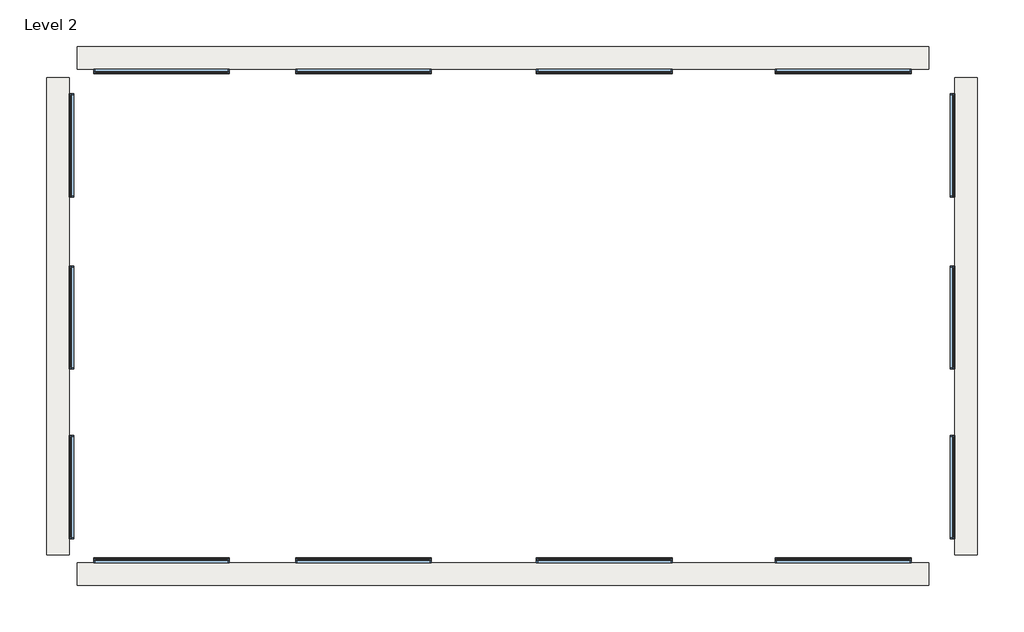
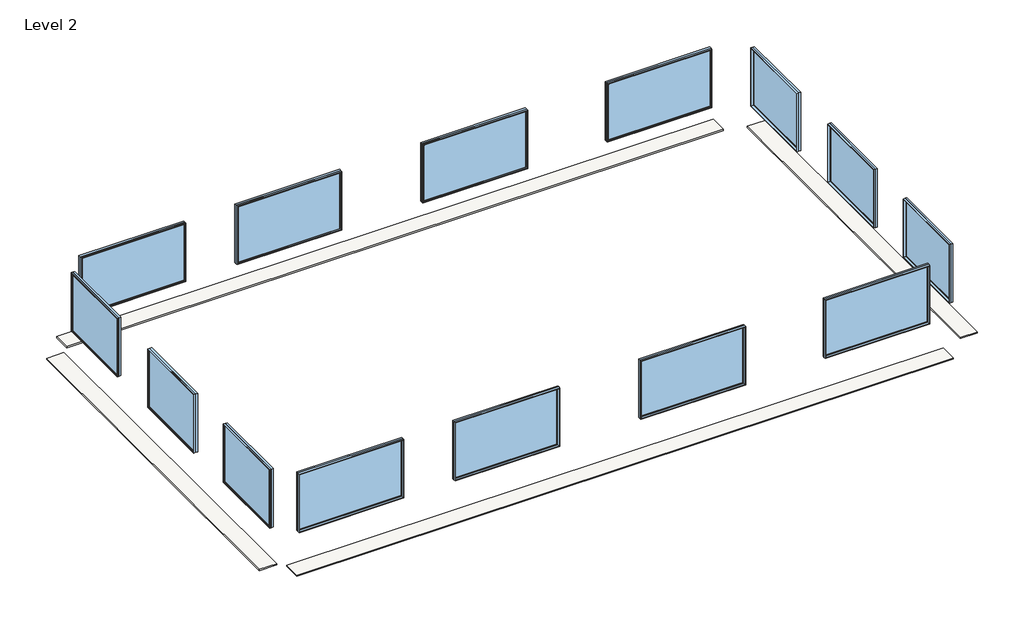
# One storey: 14 windows, 4 roofs.
"""IFC4 building model written with IfcOpenShell, lengths in millimetres."""

import ifcopenshell
import ifcopenshell.guid

model = None  # the IFC model being written
_history = None  # IfcOwnerHistory: only IFC2X3 demands one
_inside = {}  # id of a spatial element -> (the spatial element, [elements in it])
_under = {}  # id of a project, library or spatial element -> (it, [spatial elements below it])
_declared = {}  # id of a project -> (the project, [libraries it declares])
_typed = {}  # id of a type object -> (the type object, [elements of that type])
_made_of = {}  # id of a material, layer set ... -> (it, [elements and type objects made of it])


def new_model(schema):
    """Start an empty IFC model of exactly this schema.

    Asked for "IFC4X3", IfcOpenShell would pick the latest addendum, in which some entities
    have other attributes; the version numbers below select the first issue.
    IFC2X3 requires an IfcOwnerHistory on every rooted entity: one is made here for all.
    """
    global model, _history
    if schema == "IFC4X3":
        model = ifcopenshell.file(schema_version=(4, 3, 0, 0))
    else:
        model = ifcopenshell.file(schema=schema)
    _inside.clear()
    _under.clear()
    _declared.clear()
    _typed.clear()
    _made_of.clear()
    _history = None
    if model.schema == "IFC2X3":
        org = make("IfcOrganization", Name="unknown")
        user = make(
            "IfcPersonAndOrganization",
            ThePerson=make("IfcPerson", FamilyName="unknown"),
            TheOrganization=org,
        )
        app = make(
            "IfcApplication",
            ApplicationDeveloper=org,
            Version="unknown",
            ApplicationFullName="unknown",
            ApplicationIdentifier="unknown",
        )
        _history = make(
            "IfcOwnerHistory",
            OwningUser=user,
            OwningApplication=app,
            ChangeAction="ADDED",
            CreationDate=0,
        )
    return model


def make(cls, **values):
    """One entity of the class cls with the attributes given. An attribute that is None is left unset."""
    return model.create_entity(
        cls, **{name: value for name, value in values.items() if value is not None}
    )


def rooted(cls, **values):
    """An entity with a GlobalId (a new one), such as an element, a storey or a relation."""
    return make(cls, GlobalId=ifcopenshell.guid.new(), OwnerHistory=_history, **values)


def si_unit(unit_type, name, prefix=None):
    """IfcSIUnit, for example si_unit("LENGTHUNIT", "METRE", prefix="MILLI")."""
    return make("IfcSIUnit", UnitType=unit_type, Prefix=prefix, Name=name)


def assignment(units):
    """IfcUnitAssignment: the units of a project."""
    return None if units is None else make("IfcUnitAssignment", Units=units)


def point(xyz):
    """IfcCartesianPoint."""
    return None if xyz is None else make("IfcCartesianPoint", Coordinates=xyz)


def direction(xyz):
    """IfcDirection."""
    return None if xyz is None else make("IfcDirection", DirectionRatios=xyz)


def frame(location, z_axis=None, x_axis=None):
    """IfcAxis2Placement3D, a coordinate frame: its origin and axes. An axis left out is left unset."""
    return make(
        "IfcAxis2Placement3D",
        Location=point(location),
        Axis=direction(z_axis),
        RefDirection=direction(x_axis),
    )


def origin():
    """The frame at (0, 0, 0) with its axes left unset."""
    return frame((0.0, 0.0, 0.0))


def place(relative_to, where):
    """IfcLocalPlacement: puts the frame where relative to a parent placement (None: the world)."""
    return make(
        "IfcLocalPlacement", PlacementRelTo=relative_to, RelativePlacement=where
    )


def context(
    kind, dimensions, precision=None, world=None, true_north=None, identifier=None
):
    """IfcGeometricRepresentationContext, for example the 3D "Model" context."""
    return make(
        "IfcGeometricRepresentationContext",
        ContextIdentifier=identifier,
        ContextType=kind,
        CoordinateSpaceDimension=dimensions,
        Precision=precision,
        WorldCoordinateSystem=world,
        TrueNorth=true_north,
    )


def project(units=None, contexts=None):
    """IfcProject with its units and contexts."""
    return rooted(
        "IfcProject",
        Name="project",
        RepresentationContexts=contexts,
        UnitsInContext=assignment(units),
    )


def spatial(cls, under=None, at=None, **own):
    """A site, building, storey or space (cls), placed at a placement, below another one or the project."""
    s = rooted(cls, ObjectPlacement=at, **own)
    if under is not None:
        _under.setdefault(under.id(), (under, []))[1].append(s)
    return s


def polyline(points):
    """IfcPolyline through the points."""
    return make("IfcPolyline", Points=[point(p) for p in points])


def outline(outer, holes=None, kind="AREA"):
    """IfcArbitraryClosedProfileDef: a profile drawn as a closed curve; with holes, ...WithVoids."""
    if holes is None:
        return make("IfcArbitraryClosedProfileDef", ProfileType=kind, OuterCurve=outer)
    return make(
        "IfcArbitraryProfileDefWithVoids",
        ProfileType=kind,
        OuterCurve=outer,
        InnerCurves=holes,
    )


def extrude(swept, where, along, depth):
    """IfcExtrudedAreaSolid: the profile swept, set in the frame where, extruded along a direction by depth."""
    return make(
        "IfcExtrudedAreaSolid",
        SweptArea=swept,
        Position=where,
        ExtrudedDirection=direction(along),
        Depth=depth,
    )


def shape(context_of_items, identifier, shape_type, items):
    """IfcShapeRepresentation: the items that make up one representation, for example the "Body"."""
    return make(
        "IfcShapeRepresentation",
        ContextOfItems=context_of_items,
        RepresentationIdentifier=identifier,
        RepresentationType=shape_type,
        Items=items,
    )


def source(mapping_origin, context_of_items, identifier, shape_type, items):
    """IfcRepresentationMap: a shape defined once, which mapped items show again and again."""
    return make(
        "IfcRepresentationMap",
        MappingOrigin=mapping_origin,
        MappedRepresentation=shape(context_of_items, identifier, shape_type, items),
    )


def transform(
    local_origin,
    x_axis=None,
    y_axis=None,
    z_axis=None,
    scale=None,
    scale2=None,
    scale3=None,
    uniform=True,
):
    """IfcCartesianTransformationOperator3D, or its non-uniform kind. x_axis, y_axis, z_axis: its Axis1, 2, 3."""
    if uniform:
        return make(
            "IfcCartesianTransformationOperator3D",
            Axis1=direction(x_axis),
            Axis2=direction(y_axis),
            LocalOrigin=point(local_origin),
            Scale=scale,
            Axis3=direction(z_axis),
        )
    return make(
        "IfcCartesianTransformationOperator3DnonUniform",
        Axis1=direction(x_axis),
        Axis2=direction(y_axis),
        LocalOrigin=point(local_origin),
        Scale=scale,
        Axis3=direction(z_axis),
        Scale2=scale2,
        Scale3=scale3,
    )


def mapped(mapping_source, mapping_target):
    """IfcMappedItem: shows the shape of a source again, moved by a transform."""
    return make(
        "IfcMappedItem", MappingSource=mapping_source, MappingTarget=mapping_target
    )


def made_of(thing, what):
    """Note that an element or type object is made of a material, layer set ...; save() writes the relation."""
    if what is not None:
        _made_of.setdefault(what.id(), (what, []))[1].append(thing)
    return thing


def element(
    cls,
    number,
    at=None,
    inside=None,
    cuts=None,
    type_object=None,
    material=None,
    context=None,
    identifier="Body",
    shape_type=None,
    held_by="IfcProductDefinitionShape",
    body=None,
    shapes=None,
    **own,
):
    """One element of the class cls, such as IfcWall. Its Tag is "e" and its number.

    at: its placement. inside: the storey or other place that contains it. cuts: it is an
    opening in that element (IfcRelVoidsElement). A single representation is given by context,
    identifier, shape_type and body (its items); several are given by shapes. held_by: the class
    of the entity that holds the representations. save() writes the other relations.
    """
    e = rooted(cls, Tag="e%d" % number, ObjectPlacement=at, **own)
    if body is not None:
        shapes = [shape(context, identifier, shape_type, body)]
    if shapes is not None:
        e.Representation = make(held_by, Representations=shapes)
    if inside is not None:
        _inside.setdefault(inside.id(), (inside, []))[1].append(e)
    if cuts is not None:
        rooted(
            "IfcRelVoidsElement", RelatingBuildingElement=cuts, RelatedOpeningElement=e
        )
    if type_object is not None:
        _typed.setdefault(type_object.id(), (type_object, []))[1].append(e)
    return made_of(e, material)


def aggregate(whole, parts):
    """IfcRelAggregates: a whole, such as a stair, and the parts it consists of."""
    return rooted("IfcRelAggregates", RelatingObject=whole, RelatedObjects=parts)


def save(model, path):
    """Write the relations noted so far, then the file.

    IfcRelAggregates (storeys below a building ...), IfcRelContainedInSpatialStructure (elements
    in a storey), IfcRelDefinesByType, IfcRelAssociatesMaterial and IfcRelDeclares: one each for
    every whole, place, type object, material and project.
    """
    for whole, parts in _under.values():
        aggregate(whole, parts)
    for where, things in _inside.values():
        rooted(
            "IfcRelContainedInSpatialStructure",
            RelatedElements=things,
            RelatingStructure=where,
        )
    for kind, things in _typed.values():
        rooted("IfcRelDefinesByType", RelatedObjects=things, RelatingType=kind)
    for what, things in _made_of.values():
        rooted("IfcRelAssociatesMaterial", RelatedObjects=things, RelatingMaterial=what)
    for by, libraries in _declared.values():
        rooted("IfcRelDeclares", RelatingContext=by, RelatedDefinitions=libraries)
    model.write(path)


def m_fixed_2500x_4228mm_fd5e51e7(model_context):
    return source(origin(), model_context, "Body", "SweptSolid", [
        extrude(outline(polyline([(-2050.8, 54.2), (2050.8, 54.2), (2050.8, 42.2), (-2050.8, 42.2), (-2050.8, 54.2)])), frame((0.0, 0.0, 368.0), z_axis=(0.0, 0.0, 1.0), x_axis=(1.0, 0.0, 0.0)), (0.0, 0.0, 1.0), 2374.0),
        extrude(outline(polyline([(2786.0, -2094.8), (324.0, -2094.8), (324.0, 2094.8), (2786.0, 2094.8), (2786.0, -2094.8)]), holes=[polyline([(2742.0, -2050.8), (2742.0, 2050.8), (368.0, 2050.8), (368.0, -2050.8), (2742.0, -2050.8)])]), frame((0.0, 26.2, 0.0), z_axis=(0.0, 1.0, 0.0), x_axis=(0.0, 0.0, 1.0)), (0.0, 0.0, 1.0), 44.0),
        extrude(outline(polyline([(2805.0, -2113.8), (305.0, -2113.8), (305.0, 2113.8), (2805.0, 2113.8), (2805.0, -2113.8)]), holes=[polyline([(2786.0, -2094.8), (2786.0, 2094.8), (324.0, 2094.8), (324.0, -2094.8), (2786.0, -2094.8)])]), frame((0.0, 26.2, 0.0), z_axis=(0.0, 1.0, 0.0), x_axis=(0.0, 0.0, 1.0)), (0.0, 0.0, 1.0), 63.0),
        extrude(outline(polyline([(2805.0, -2113.8), (305.0, -2113.8), (305.0, 2113.8), (2805.0, 2113.8), (2805.0, -2113.8)]), holes=[polyline([(2773.0, -2081.8), (2773.0, 2081.8), (337.0, 2081.8), (337.0, -2081.8), (2773.0, -2081.8)])]), frame((0.0, -63.2, 0.0), z_axis=(0.0, 1.0, 0.0), x_axis=(0.0, 0.0, 1.0)), (0.0, 0.0, 1.0), 89.4),
    ])


def m_fixed_2500x_4228mm_f14c179f(model_context):
    return source(origin(), model_context, "Body", "SweptSolid", [
        extrude(outline(polyline([(-2050.8, -54.2), (-2050.8, -42.2), (2050.8, -42.2), (2050.8, -54.2), (-2050.8, -54.2)])), frame((0.0, 0.0, 368.0), z_axis=(0.0, 0.0, 1.0), x_axis=(1.0, 0.0, 0.0)), (0.0, 0.0, 1.0), 2374.0),
        extrude(outline(polyline([(2786.0, -2094.8), (324.0, -2094.8), (324.0, 2094.8), (2786.0, 2094.8), (2786.0, -2094.8)]), holes=[polyline([(2742.0, -2050.8), (2742.0, 2050.8), (368.0, 2050.8), (368.0, -2050.8), (2742.0, -2050.8)])]), frame((0.0, -70.2, 0.0), z_axis=(0.0, 1.0, 0.0), x_axis=(0.0, 0.0, 1.0)), (0.0, 0.0, 1.0), 44.0),
        extrude(outline(polyline([(2805.0, -2113.8), (305.0, -2113.8), (305.0, 2113.8), (2805.0, 2113.8), (2805.0, -2113.8)]), holes=[polyline([(2786.0, -2094.8), (2786.0, 2094.8), (324.0, 2094.8), (324.0, -2094.8), (2786.0, -2094.8)])]), frame((0.0, -89.2, 0.0), z_axis=(0.0, 1.0, 0.0), x_axis=(0.0, 0.0, 1.0)), (0.0, 0.0, 1.0), 63.0),
        extrude(outline(polyline([(2805.0, -2113.8), (305.0, -2113.8), (305.0, 2113.8), (2805.0, 2113.8), (2805.0, -2113.8)]), holes=[polyline([(2773.0, -2081.8), (2773.0, 2081.8), (337.0, 2081.8), (337.0, -2081.8), (2773.0, -2081.8)])]), frame((0.0, -26.2, 0.0), z_axis=(0.0, 1.0, 0.0), x_axis=(0.0, 0.0, 1.0)), (0.0, 0.0, 1.0), 89.4),
    ])


def m_fixed_2500x_3220mm_df94f4d0(model_context):
    return source(origin(), model_context, "Body", "SweptSolid", [
        extrude(outline(polyline([(-1546.8, 54.2), (1546.8, 54.2), (1546.8, 42.2), (-1546.8, 42.2), (-1546.8, 54.2)])), frame((0.0, 0.0, 368.0), z_axis=(0.0, 0.0, 1.0), x_axis=(1.0, 0.0, 0.0)), (0.0, 0.0, 1.0), 2374.0),
        extrude(outline(polyline([(2786.0, -1590.8), (324.0, -1590.8), (324.0, 1590.8), (2786.0, 1590.8), (2786.0, -1590.8)]), holes=[polyline([(2742.0, -1546.8), (2742.0, 1546.8), (368.0, 1546.8), (368.0, -1546.8), (2742.0, -1546.8)])]), frame((0.0, 26.2, 0.0), z_axis=(0.0, 1.0, 0.0), x_axis=(0.0, 0.0, 1.0)), (0.0, 0.0, 1.0), 44.0),
        extrude(outline(polyline([(2805.0, -1609.8), (305.0, -1609.8), (305.0, 1609.8), (2805.0, 1609.8), (2805.0, -1609.8)]), holes=[polyline([(2786.0, -1590.8), (2786.0, 1590.8), (324.0, 1590.8), (324.0, -1590.8), (2786.0, -1590.8)])]), frame((0.0, 26.2, 0.0), z_axis=(0.0, 1.0, 0.0), x_axis=(0.0, 0.0, 1.0)), (0.0, 0.0, 1.0), 63.0),
        extrude(outline(polyline([(2805.0, -1609.8), (305.0, -1609.8), (305.0, 1609.8), (2805.0, 1609.8), (2805.0, -1609.8)]), holes=[polyline([(2773.0, -1577.8), (2773.0, 1577.8), (337.0, 1577.8), (337.0, -1577.8), (2773.0, -1577.8)])]), frame((0.0, -63.2, 0.0), z_axis=(0.0, 1.0, 0.0), x_axis=(0.0, 0.0, 1.0)), (0.0, 0.0, 1.0), 89.4),
    ])


def m_fixed_2500x_3220mm_8b997f8c(model_context):
    return source(origin(), model_context, "Body", "SweptSolid", [
        extrude(outline(polyline([(-1546.8, -54.2), (-1546.8, -42.2), (1546.8, -42.2), (1546.8, -54.2), (-1546.8, -54.2)])), frame((0.0, 0.0, 368.0), z_axis=(0.0, 0.0, 1.0), x_axis=(1.0, 0.0, 0.0)), (0.0, 0.0, 1.0), 2374.0),
        extrude(outline(polyline([(2786.0, -1590.8), (324.0, -1590.8), (324.0, 1590.8), (2786.0, 1590.8), (2786.0, -1590.8)]), holes=[polyline([(2742.0, -1546.8), (2742.0, 1546.8), (368.0, 1546.8), (368.0, -1546.8), (2742.0, -1546.8)])]), frame((0.0, -70.2, 0.0), z_axis=(0.0, 1.0, 0.0), x_axis=(0.0, 0.0, 1.0)), (0.0, 0.0, 1.0), 44.0),
        extrude(outline(polyline([(2805.0, -1609.8), (305.0, -1609.8), (305.0, 1609.8), (2805.0, 1609.8), (2805.0, -1609.8)]), holes=[polyline([(2786.0, -1590.8), (2786.0, 1590.8), (324.0, 1590.8), (324.0, -1590.8), (2786.0, -1590.8)])]), frame((0.0, -89.2, 0.0), z_axis=(0.0, 1.0, 0.0), x_axis=(0.0, 0.0, 1.0)), (0.0, 0.0, 1.0), 63.0),
        extrude(outline(polyline([(2805.0, -1609.8), (305.0, -1609.8), (305.0, 1609.8), (2805.0, 1609.8), (2805.0, -1609.8)]), holes=[polyline([(2773.0, -1577.8), (2773.0, 1577.8), (337.0, 1577.8), (337.0, -1577.8), (2773.0, -1577.8)])]), frame((0.0, -26.2, 0.0), z_axis=(0.0, 1.0, 0.0), x_axis=(0.0, 0.0, 1.0)), (0.0, 0.0, 1.0), 89.4),
    ])


model = new_model("IFC4")

# Units and contexts
model_context = context("Model", 3, world=origin())
ifc_project = project(units=[si_unit("LENGTHUNIT", "METRE", prefix="MILLI")], contexts=[model_context])

# Site, building, storey
site = spatial("IfcSite", under=ifc_project)
building = spatial("IfcBuilding", under=site)
storey = spatial("IfcBuildingStorey", under=building, Name="Level 2", Elevation=3962.4)

# Roofs
placement = place(None, origin())
element("IfcRoof", 1, ObjectType="Shading devices - 50mm", at=placement, inside=storey, context=model_context, shape_type="SweptSolid", body=[
    extrude(outline(polyline([(1746.464681, -4095.4197783), (28246.464681, -4095.4197783), (28246.464681, -4795.4197783), (1746.464681, -4795.4197783), (1746.464681, -4095.4197783)])), frame((0.0, 0.0, 3602.4), z_axis=(0.0, 0.0, 1.0), x_axis=(1.0, 0.0, 0.0)), (0.0, 0.0, 1.0), 50.0),
])
element("IfcRoof", 2, ObjectType="Shading devices - 50mm", at=placement, inside=storey, context=model_context, shape_type="SweptSolid", body=[
    extrude(outline(polyline([(29068.464681, 11030.5802217), (29768.464681, 11030.5802217), (29768.464681, -3843.0197783), (29068.464681, -3843.0197783), (29068.464681, 11030.5802217)])), frame((0.0, 0.0, 3602.4), z_axis=(0.0, 0.0, 1.0), x_axis=(1.0, 0.0, 0.0)), (0.0, 0.0, 1.0), 50.0),
])
element("IfcRoof", 3, ObjectType="Shading devices - 50mm", at=placement, inside=storey, context=model_context, shape_type="SweptSolid", body=[
    extrude(outline(polyline([(28246.464681, 11296.9802217), (1746.464681, 11296.9802217), (1746.464681, 11996.9802217), (28246.464681, 11996.9802217), (28246.464681, 11296.9802217)])), frame((0.0, 0.0, 3602.4), z_axis=(0.0, 0.0, 1.0), x_axis=(1.0, 0.0, 0.0)), (0.0, 0.0, 1.0), 50.0),
])
element("IfcRoof", 4, ObjectType="Shading devices - 50mm", at=placement, inside=storey, context=model_context, shape_type="SweptSolid", body=[
    extrude(outline(polyline([(784.064681, 11030.5802217), (1484.064681, 11030.5802217), (1484.064681, -3843.0197783), (784.064681, -3843.0197783), (784.064681, 11030.5802217)])), frame((0.0, 0.0, 3602.4), z_axis=(0.0, 0.0, 1.0), x_axis=(1.0, 0.0, 0.0)), (0.0, 0.0, 1.0), 50.0),
])

# Windows
m_fixed_2500x_4228mm_shape = m_fixed_2500x_4228mm_fd5e51e7(model_context)
element("IfcWindow", 5, ObjectType="M_Fixed : 2500X 4228mm", at=placement, inside=storey, context=model_context, shape_type="MappedRepresentation", body=[
    mapped(m_fixed_2500x_4228mm_shape, transform((4360.264681, 11233.7802217, 4557.4), x_axis=(-1.0, 0.0, 0.0), y_axis=(0.0, -1.0, 0.0), z_axis=(0.0, 0.0, 1.0))),
])
element("IfcWindow", 6, ObjectType="M_Fixed : 2500X 4228mm", at=placement, inside=storey, context=model_context, shape_type="MappedRepresentation", body=[
    mapped(m_fixed_2500x_4228mm_shape, transform((10652.264681, 11233.7802217, 4557.4), x_axis=(-1.0, 0.0, 0.0), y_axis=(0.0, -1.0, 0.0), z_axis=(0.0, 0.0, 1.0))),
])
element("IfcWindow", 7, ObjectType="M_Fixed : 2500X 4228mm", at=placement, inside=storey, context=model_context, shape_type="MappedRepresentation", body=[
    mapped(m_fixed_2500x_4228mm_shape, transform((18152.264681, 11233.7802217, 4557.4), x_axis=(-1.0, 0.0, 0.0), y_axis=(0.0, -1.0, 0.0), z_axis=(0.0, 0.0, 1.0))),
])
element("IfcWindow", 8, ObjectType="M_Fixed : 2500X 4228mm", at=placement, inside=storey, context=model_context, shape_type="MappedRepresentation", body=[
    mapped(m_fixed_2500x_4228mm_shape, transform((25592.264681, 11233.7802217, 4557.4), x_axis=(-1.0, 0.0, 0.0), y_axis=(0.0, -1.0, 0.0), z_axis=(0.0, 0.0, 1.0))),
])
m_fixed_2500x_4228mm_2_shape = m_fixed_2500x_4228mm_f14c179f(model_context)
element("IfcWindow", 9, ObjectType="M_Fixed : 2500X 4228mm", at=placement, inside=storey, context=model_context, shape_type="MappedRepresentation", body=[
    mapped(m_fixed_2500x_4228mm_2_shape, transform((4360.264681, -4032.2197783, 4557.4), x_axis=(-1.0, 0.0, 0.0), y_axis=(0.0, -1.0, 0.0), z_axis=(0.0, 0.0, 1.0))),
])
element("IfcWindow", 10, ObjectType="M_Fixed : 2500X 4228mm", at=placement, inside=storey, context=model_context, shape_type="MappedRepresentation", body=[
    mapped(m_fixed_2500x_4228mm_2_shape, transform((10652.264681, -4032.2197783, 4557.4), x_axis=(-1.0, 0.0, 0.0), y_axis=(0.0, -1.0, 0.0), z_axis=(0.0, 0.0, 1.0))),
])
element("IfcWindow", 11, ObjectType="M_Fixed : 2500X 4228mm", at=placement, inside=storey, context=model_context, shape_type="MappedRepresentation", body=[
    mapped(m_fixed_2500x_4228mm_2_shape, transform((18152.264681, -4032.2197783, 4557.4), x_axis=(-1.0, 0.0, 0.0), y_axis=(0.0, -1.0, 0.0), z_axis=(0.0, 0.0, 1.0))),
])
element("IfcWindow", 12, ObjectType="M_Fixed : 2500X 4228mm", at=placement, inside=storey, context=model_context, shape_type="MappedRepresentation", body=[
    mapped(m_fixed_2500x_4228mm_2_shape, transform((25592.264681, -4032.2197783, 4557.4), x_axis=(-1.0, 0.0, 0.0), y_axis=(0.0, -1.0, 0.0), z_axis=(0.0, 0.0, 1.0))),
])
m_fixed_2500x_3220mm_shape = m_fixed_2500x_3220mm_df94f4d0(model_context)
element("IfcWindow", 13, ObjectType="M_Fixed : 2500x 3220mm", at=placement, inside=storey, context=model_context, shape_type="MappedRepresentation", body=[
    mapped(m_fixed_2500x_3220mm_shape, transform((1573.264681, 8920.7802217, 4559.8), x_axis=(0.0, 1.0, 0.0), y_axis=(-1.0, 0.0, 0.0), z_axis=(0.0, 0.0, 1.0))),
])
element("IfcWindow", 14, ObjectType="M_Fixed : 2500x 3220mm", at=placement, inside=storey, context=model_context, shape_type="MappedRepresentation", body=[
    mapped(m_fixed_2500x_3220mm_shape, transform((1573.264681, 3552.7802217, 4559.8), x_axis=(0.0, 1.0, 0.0), y_axis=(-1.0, 0.0, 0.0), z_axis=(0.0, 0.0, 1.0))),
])
element("IfcWindow", 15, ObjectType="M_Fixed : 2500x 3220mm", at=placement, inside=storey, context=model_context, shape_type="MappedRepresentation", body=[
    mapped(m_fixed_2500x_3220mm_shape, transform((1573.264681, -1733.2197783, 4559.8), x_axis=(0.0, 1.0, 0.0), y_axis=(-1.0, 0.0, 0.0), z_axis=(0.0, 0.0, 1.0))),
])
m_fixed_2500x_3220mm_2_shape = m_fixed_2500x_3220mm_8b997f8c(model_context)
element("IfcWindow", 16, ObjectType="M_Fixed : 2500x 3220mm", at=placement, inside=storey, context=model_context, shape_type="MappedRepresentation", body=[
    mapped(m_fixed_2500x_3220mm_2_shape, transform((28979.264681, 8920.7802217, 4559.8), x_axis=(0.0, 1.0, 0.0), y_axis=(-1.0, 0.0, 0.0), z_axis=(0.0, 0.0, 1.0))),
])
element("IfcWindow", 17, ObjectType="M_Fixed : 2500x 3220mm", at=placement, inside=storey, context=model_context, shape_type="MappedRepresentation", body=[
    mapped(m_fixed_2500x_3220mm_2_shape, transform((28979.264681, 3552.7802217, 4559.8), x_axis=(0.0, 1.0, 0.0), y_axis=(-1.0, 0.0, 0.0), z_axis=(0.0, 0.0, 1.0))),
])
element("IfcWindow", 18, ObjectType="M_Fixed : 2500x 3220mm", at=placement, inside=storey, context=model_context, shape_type="MappedRepresentation", body=[
    mapped(m_fixed_2500x_3220mm_2_shape, transform((28979.264681, -1733.2197783, 4559.8), x_axis=(0.0, 1.0, 0.0), y_axis=(-1.0, 0.0, 0.0), z_axis=(0.0, 0.0, 1.0))),
])

save(model, "model.ifc")

# Revit data of these elements
# Project information
#   Project Issue Date = "Issue Date"
#   Project Status = "Project Status"
#   Client Name = "Owner"
#   Project Address = "Enter address here"
#   Project Name = "Project Name"
#   Project Number = "Project Number"
# Type "Shading devices - 50mm"
#   Layers, outside or top first: 50 mm no material (function 1)
# Type "M_Fixed : 2500X 4228mm"
#   Type Mark = "25"
#   Height = 2500 mm
#   Default Sill Height = 305 mm
#   Width = 4227.6 mm
#   Window Inset = 19 mm
#   Frame Exterior Material = Sash
#   Frame Interior Material = Sash
#   Glass Pane Material = Glass
#   Sash = Sash
#   Wall Closure = (empty or 0)
# Type "M_Fixed : 2500x 3220mm"
#   Type Mark = "26"
#   Height = 2500 mm
#   Default Sill Height = 305 mm
#   Width = 3219.6 mm
#   Window Inset = 19 mm
#   Frame Exterior Material = Sash
#   Frame Interior Material = Sash
#   Glass Pane Material = Glass
#   Sash = Sash
#   Wall Closure = (empty or 0)
# Elements 1, 2, 3, 4 (IfcRoof, "Shading devices - 50mm")
#   built-in parameter 1001705 = 11.9829 (stored number, unit not read)
#   built-in parameter 1001701 = -1.1811 (stored number, unit not read)
#   built-in parameter 1001710 = 33615
#   Phase Created = New Construction
#   Materials on its faces: "Default Roof"
# Element 5 (IfcWindow, "M_Fixed : 2500X 4228mm")
#   Mark = "1"
#   Phase Created = New Construction
#   Materials on its faces: "Sash", "Glass"
# Element 6 (IfcWindow, "M_Fixed : 2500X 4228mm")
#   Mark = "2"
#   Phase Created = New Construction
#   Materials on its faces: "Sash", "Glass"
# Element 7 (IfcWindow, "M_Fixed : 2500X 4228mm")
#   Mark = "3"
#   Phase Created = New Construction
#   Materials on its faces: "Sash", "Glass"
# Element 8 (IfcWindow, "M_Fixed : 2500X 4228mm")
#   Mark = "4"
#   Phase Created = New Construction
#   Materials on its faces: "Sash", "Glass"
# Element 9 (IfcWindow, "M_Fixed : 2500X 4228mm")
#   Mark = "5"
#   Phase Created = New Construction
#   Materials on its faces: "Sash", "Glass"
# Element 10 (IfcWindow, "M_Fixed : 2500X 4228mm")
#   Mark = "6"
#   Phase Created = New Construction
#   Materials on its faces: "Sash", "Glass"
# Element 11 (IfcWindow, "M_Fixed : 2500X 4228mm")
#   Mark = "7"
#   Phase Created = New Construction
#   Materials on its faces: "Sash", "Glass"
# Element 12 (IfcWindow, "M_Fixed : 2500X 4228mm")
#   Mark = "8"
#   Phase Created = New Construction
#   Materials on its faces: "Sash", "Glass"
# Element 13 (IfcWindow, "M_Fixed : 2500x 3220mm")
#   Mark = "29"
#   Phase Created = New Construction
#   Materials on its faces: "Sash", "Glass"
# Element 14 (IfcWindow, "M_Fixed : 2500x 3220mm")
#   Mark = "33"
#   Phase Created = New Construction
#   Materials on its faces: "Sash", "Glass"
# Element 15 (IfcWindow, "M_Fixed : 2500x 3220mm")
#   Mark = "34"
#   Phase Created = New Construction
#   Materials on its faces: "Sash", "Glass"
# Element 16 (IfcWindow, "M_Fixed : 2500x 3220mm")
#   Mark = "20"
#   Phase Created = New Construction
#   Materials on its faces: "Sash", "Glass"
# Element 17 (IfcWindow, "M_Fixed : 2500x 3220mm")
#   Mark = "21"
#   Phase Created = New Construction
#   Materials on its faces: "Sash", "Glass"
# Element 18 (IfcWindow, "M_Fixed : 2500x 3220mm")
#   Mark = "22"
#   Phase Created = New Construction
#   Materials on its faces: "Sash", "Glass"
# Materials
#   "Sash": class "Wood", colour RGB 136 99 55, transparency 0
#   "Glass": class "Glass", colour RGB 0 128 192, transparency 0.9, Description = "Soda Lime Glass", Cost = 0
#   "Default Roof": class "Miscellaneous", colour RGB 0 127 0, transparency 0, Cost = 0
# Space at (4981.601, 8740.056) mm, phase "New Construction", upper level "Level 2", upper offset 3962.4 mm, lower offset 0 mm
#   Number = "5"
#   Name = "Space"
#   Actual Lighting Load per area = 0
#   Actual Power Load per area = 0
#   Sensible Heat Gain per person = 0
#   Specified Lighting Load = 6165.03 (stored number, unit not read)
#   Specified Power Load = 8014.54 (stored number, unit not read)
#   Latent Heat Gain per person = 0
#   Total Heat Gain per person = 0
#   Area per Person = 0
#   Number of People = 1.86236 (stored number, unit not read)
#   Lighting Load Units = 0
#   Power Load Units = 0
#   Return Airflow = 0
#   Occupancy Unit = -1
#   Condition Type = 1
#   Construction Type = none
# Space at (7636.211, 2935.909) mm, phase "New Construction", upper level "Level 2", upper offset 3962.4 mm, lower offset 0 mm
#   Number = "6"
#   Name = "Space"
#   Actual Lighting Load per area = 0
#   Actual Power Load per area = 0
#   Sensible Heat Gain per person = 0
#   Specified Lighting Load = 14668.5 (stored number, unit not read)
#   Specified Power Load = 19069.1 (stored number, unit not read)
#   Latent Heat Gain per person = 0
#   Total Heat Gain per person = 0
#   Area per Person = 0
#   Number of People = 4.43113 (stored number, unit not read)
#   Lighting Load Units = 0
#   Power Load Units = 0
#   Return Airflow = 0
#   Occupancy Unit = -1
#   Condition Type = 1
#   Construction Type = none
# Room at (7702.307, 8283.876) mm, phase "New Construction", upper level "Roof Level", upper offset 0 mm, lower offset 0 mm
#   Number = "9"
#   Name = "Room"
# Room at (8641.307, 981.272) mm, phase "New Construction", upper level "Roof Level", upper offset 0 mm, lower offset 0 mm
#   Number = "10"
#   Name = "Room"
